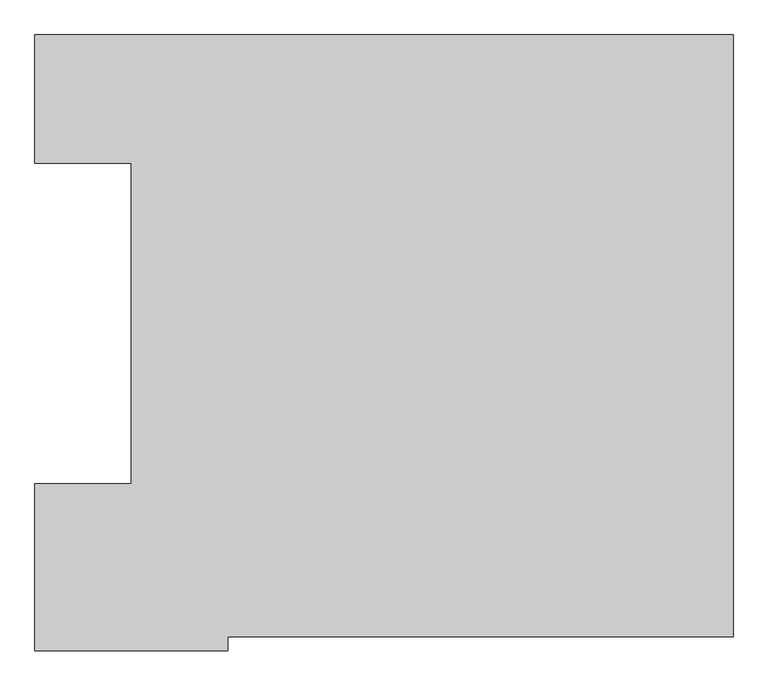
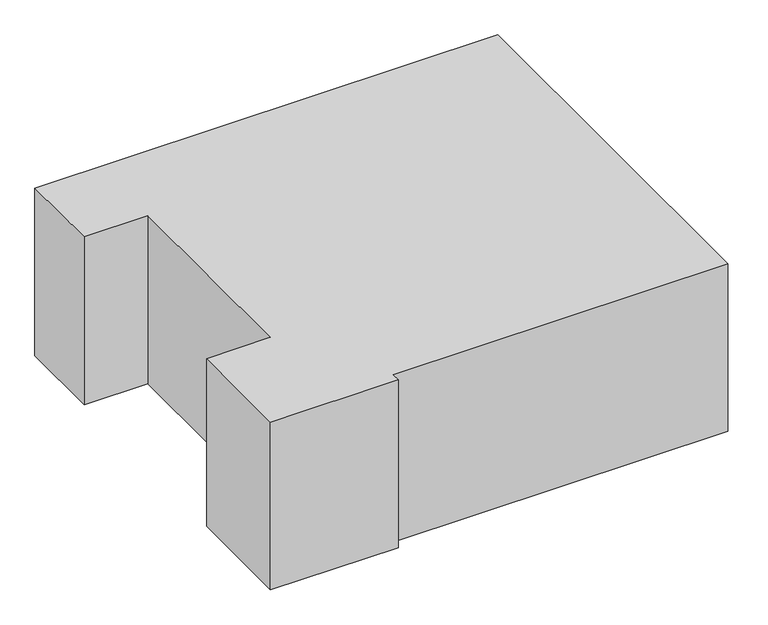
"""IFC4 building model written with IfcOpenShell, lengths in millimetres: proxy geometry, 0_3d."""

from ifc_helpers import new_model, si_unit, origin, origin_with_axes, place, context, project, spatial, polyline, outline, extrude, source, transform, mapped, element, save


def generic_models_10512bfc(model_context):
    return source(origin(), model_context, "Body", "SweptSolid", [
        extrude(outline(polyline([(0.0, 0.0), (0.0, 1560.0), (900.0, 1560.0), (900.0, 4550.0), (0.0, 4550.0), (0.0, 5750.0), (6520.0, 5750.0), (6520.0, 130.0), (1800.0, 130.0), (1800.0, 0.0), (0.0, 0.0)])), origin_with_axes(), (0.0, 0.0, 1.0), 2500.0),
    ])


if __name__ == "__main__":
    model = new_model("IFC4")
    model_context = context("Model", 3, world=origin())
    ifc_project = project(units=[si_unit("LENGTHUNIT", "METRE", prefix="MILLI")], contexts=[model_context])
    site = spatial("IfcSite", under=ifc_project)
    building = spatial("IfcBuilding", under=site)
    placement = place(None, origin())
    generic_models_shape = generic_models_10512bfc(model_context)
    element("IfcBuildingElementProxy", 1, Name="0_3d", ObjectType="0_3d", at=placement, inside=building, context=model_context, shape_type="MappedRepresentation", body=[
        mapped(generic_models_shape, transform((0.0, 0.0, 0.0), x_axis=(1.0, 0.0, 0.0), y_axis=(0.0, 1.0, 0.0), z_axis=(0.0, 0.0, 1.0))),
    ])
    save(model, "model.ifc")

# Revit data of these elements
# Element 1 (IfcBuildingElementProxy, "0_3d")
#   Materials on its faces: "*1"
# Materials
#   "*1": class "Unassigned", colour RGB 175 175 175, transparency 0
